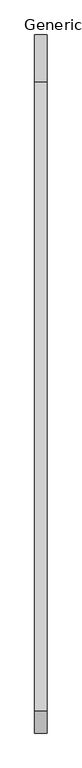
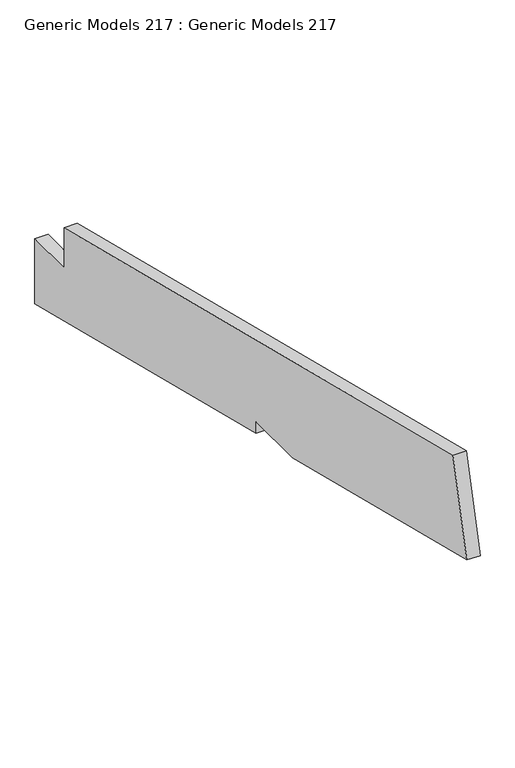
"""IFC4 building model written with IfcOpenShell, lengths in millimetres: proxy geometry, Generic Models 217 : Generic Models 217."""

from ifc_helpers import new_model, si_unit, frame, origin, place, context, project, spatial, polyline, outline, extrude, source, transform, mapped, element, save


def generic_models_217_generic_models_217_8069ab4e(model_context):
    return source(origin(), model_context, "Body", "SweptSolid", [
        extrude(outline(polyline([(12445.4269662, 129598.5345789), (12445.4269662, 129476.4447278), (12591.4769662, 129476.4447278), (12591.4769662, 129279.5947278), (11487.9215842, 129554.7419873), (11487.9215842, 129588.5459747), (11307.2039504, 129588.5459747), (10436.5236638, 129806.2160463), (10505.8282187, 130083.4342657), (12445.4269662, 129598.5345789)])), frame((1065.7410488, 0.0, 0.0), z_axis=(1.0, 0.0, 0.0), x_axis=(0.0, 1.0, 0.0)), (0.0, 0.0, 1.0), 38.1),
    ])


if __name__ == "__main__":
    model = new_model("IFC4")
    model_context = context("Model", 3, world=origin())
    ifc_project = project(units=[si_unit("LENGTHUNIT", "METRE", prefix="MILLI")], contexts=[model_context])
    site = spatial("IfcSite", under=ifc_project)
    building = spatial("IfcBuilding", under=site)
    placement = place(None, origin())
    generic_models_217_generic_models_217_shape = generic_models_217_generic_models_217_8069ab4e(model_context)
    element("IfcBuildingElementProxy", 1, Name="Generic Models 217 : Generic Models 217", ObjectType="Generic Models 217 : Generic Models 217", at=placement, inside=building, context=model_context, shape_type="MappedRepresentation", body=[
        mapped(generic_models_217_generic_models_217_shape, transform((0.0, 0.0, 0.0), x_axis=(1.0, 0.0, 0.0), y_axis=(0.0, 1.0, 0.0), z_axis=(0.0, 0.0, 1.0))),
    ])
    save(model, "model.ifc")

# Revit data of these elements
# Element 1 (IfcBuildingElementProxy, "Generic Models 217 : Generic Models 217")
#   Materials on its faces: "_STRUCTURAL MEMBER (SEE STRUCT. DWGS)"
# Materials
#   "_STRUCTURAL MEMBER (SEE STRUCT. DWGS)": class "Generic", colour RGB 209 182 141, transparency 0, Cost = 0
